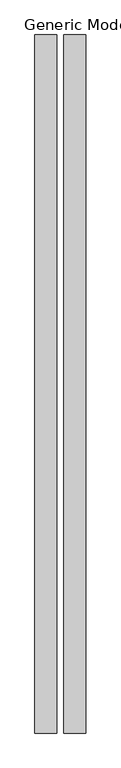
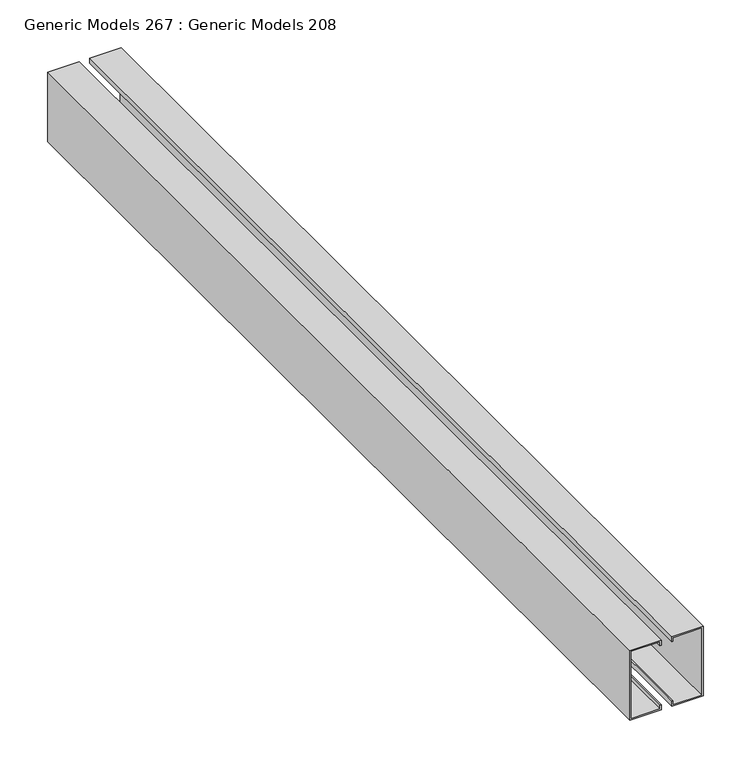
"""IFC4 building model written with IfcOpenShell, lengths in millimetres: proxy geometry, Generic Models 267 : Generic Models 208."""

from ifc_helpers import new_model, si_unit, frame, origin, place, context, project, spatial, polyline, outline, extrude, source, transform, mapped, element, save


def generic_models_267_generic_models_208_66f8256b(model_context):
    return source(origin(), model_context, "Body", "SweptSolid", [
        extrude(outline(polyline([(2168.128125, 55718.8454676), (2163.365625, 55718.8454676), (2163.365625, 55720.4329676), (2169.715625, 55720.4329676), (2169.715625, 55682.3329676), (2080.815625, 55682.3329676), (2080.815625, 55720.4329676), (2087.165625, 55720.4329676), (2087.165625, 55718.8454676), (2082.403125, 55718.8454676), (2082.403125, 55683.9204676), (2168.128125, 55683.9204676), (2168.128125, 55718.8454676)])), frame((0.0, -228.7033818, 0.0), z_axis=(0.0, 1.0, 0.0), x_axis=(0.0, 0.0, 1.0)), (0.0, 0.0, 1.0), 1219.2),
        extrude(outline(polyline([(2168.128125, 55734.7204676), (2168.128125, 55769.6454676), (2082.403125, 55769.6454676), (2082.403125, 55734.7204676), (2087.165625, 55734.7204676), (2087.165625, 55733.1329676), (2080.815625, 55733.1329676), (2080.815625, 55771.2329676), (2169.715625, 55771.2329676), (2169.715625, 55733.1329676), (2163.365625, 55733.1329676), (2163.365625, 55734.7204676), (2168.128125, 55734.7204676)])), frame((0.0, -228.7033818, 0.0), z_axis=(0.0, 1.0, 0.0), x_axis=(0.0, 0.0, 1.0)), (0.0, 0.0, 1.0), 1219.2),
    ])


if __name__ == "__main__":
    model = new_model("IFC4")
    model_context = context("Model", 3, world=origin())
    ifc_project = project(units=[si_unit("LENGTHUNIT", "METRE", prefix="MILLI")], contexts=[model_context])
    site = spatial("IfcSite", under=ifc_project)
    building = spatial("IfcBuilding", under=site)
    placement = place(None, origin())
    generic_models_267_generic_models_208_shape = generic_models_267_generic_models_208_66f8256b(model_context)
    element("IfcBuildingElementProxy", 1, Name="Generic Models 267 : Generic Models 208", ObjectType="Generic Models 267 : Generic Models 208", at=placement, inside=building, context=model_context, shape_type="MappedRepresentation", body=[
        mapped(generic_models_267_generic_models_208_shape, transform((0.0, 0.0, 0.0), x_axis=(1.0, 0.0, 0.0), y_axis=(0.0, 1.0, 0.0), z_axis=(0.0, 0.0, 1.0))),
    ])
    save(model, "model.ifc")

# Revit data of these elements
# Element 1 (IfcBuildingElementProxy, "Generic Models 267 : Generic Models 208")
#   Materials on its faces: "METAL STUD"
# Materials
#   "METAL STUD": class "Metal", colour RGB 244 244 244, transparency 0, Description = "Aluminum 6061", Cost = 0
